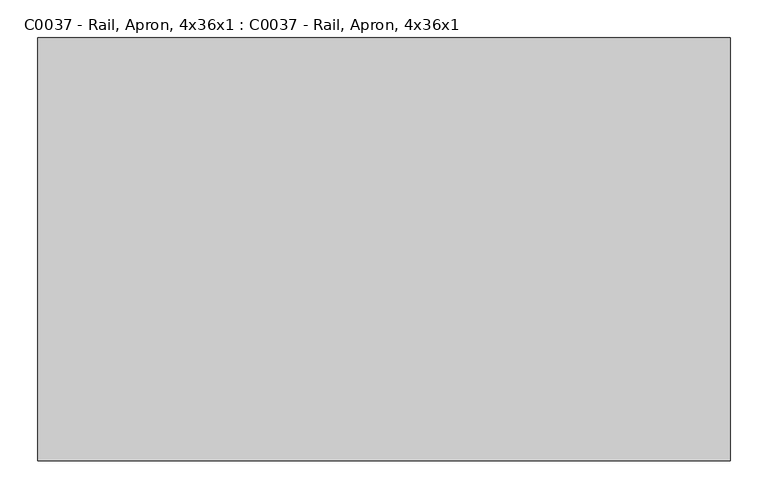
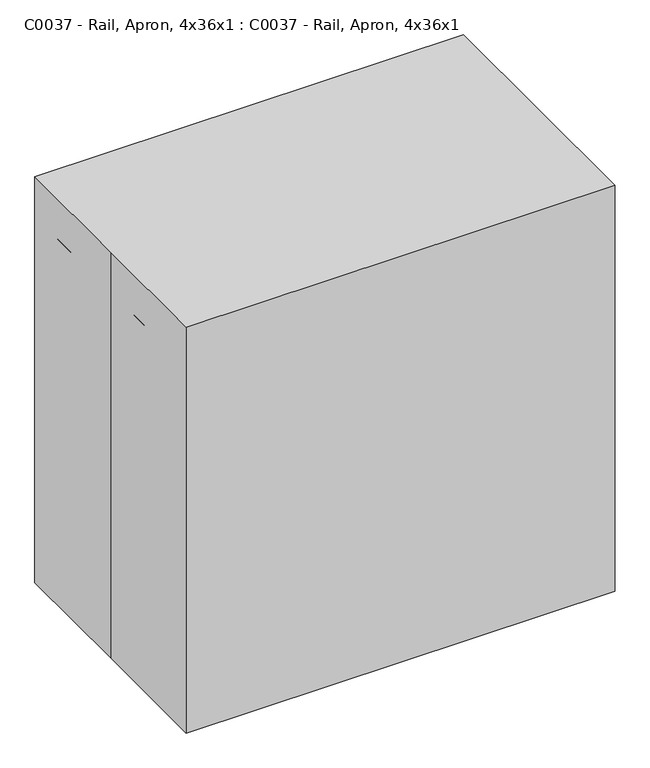
"""IFC4 building model written with IfcOpenShell, lengths in millimetres: proxy geometry, C0037 - Rail, Apron, 4x36x1 : C0037 - Rail, Apron, 4x36x1."""

from ifc_helpers import new_model, si_unit, frame, origin, origin_with_axes, place, context, project, spatial, polyline, outline, extrude, source, transform, mapped, element, save


def c0037_rail_apron_4x36x1_c0037_rail_apron_4x36x1_112512d8(model_context):
    return source(origin(), model_context, "Body", "SweptSolid", [
        extrude(outline(polyline([(-457.2, 279.4), (457.2, 279.4), (457.2, -279.4), (-457.2, -279.4), (-457.2, 0.0), (-457.2, 279.4)])), origin_with_axes(), (0.0, 0.0, 1.0), 914.4),
        extrude(outline(polyline([(438.15, -260.35), (438.15, 279.4), (457.2, 279.4), (457.2, -260.35), (438.15, -260.35)])), frame((0.0, 0.0, 673.0674767), z_axis=(0.0, 0.0, 1.0), x_axis=(1.0, 0.0, 0.0)), (0.0, 0.0, 1.0), 152.4),
        extrude(outline(polyline([(-457.2, -260.35), (-457.2, 279.4), (-438.15, 279.4), (-438.15, -260.35), (-457.2, -260.35)])), frame((0.0, 0.0, 673.0674767), z_axis=(0.0, 0.0, 1.0), x_axis=(1.0, 0.0, 0.0)), (0.0, 0.0, 1.0), 152.4),
        extrude(outline(polyline([(457.2, -279.4), (-457.2, -279.4), (-457.2, -260.35), (457.2, -260.35), (457.2, -279.4)])), frame((0.0, 0.0, 673.0674767), z_axis=(0.0, 0.0, 1.0), x_axis=(1.0, 0.0, 0.0)), (0.0, 0.0, 1.0), 152.4),
        extrude(outline(polyline([(438.15, 260.35), (-438.15, 260.35), (-438.15, 279.4), (438.15, 279.4), (438.15, 260.35)])), frame((0.0, 0.0, 673.0674767), z_axis=(0.0, 0.0, 1.0), x_axis=(1.0, 0.0, 0.0)), (0.0, 0.0, 1.0), 133.35),
    ])


if __name__ == "__main__":
    model = new_model("IFC4")
    model_context = context("Model", 3, world=origin())
    ifc_project = project(units=[si_unit("LENGTHUNIT", "METRE", prefix="MILLI")], contexts=[model_context])
    site = spatial("IfcSite", under=ifc_project)
    building = spatial("IfcBuilding", under=site)
    placement = place(None, origin())
    c0037_rail_apron_4x36x1_c0037_rail_apron_4x36x1_shape = c0037_rail_apron_4x36x1_c0037_rail_apron_4x36x1_112512d8(model_context)
    element("IfcBuildingElementProxy", 1, Name="C0037 - Rail, Apron, 4x36x1 : C0037 - Rail, Apron, 4x36x1", ObjectType="C0037 - Rail, Apron, 4x36x1 : C0037 - Rail, Apron, 4x36x1", at=placement, inside=building, context=model_context, shape_type="MappedRepresentation", body=[
        mapped(c0037_rail_apron_4x36x1_c0037_rail_apron_4x36x1_shape, transform((0.0, 0.0, 0.0), x_axis=(1.0, 0.0, 0.0), y_axis=(0.0, 1.0, 0.0), z_axis=(0.0, 0.0, 1.0))),
    ])
    save(model, "model.ifc")

# Revit data of these elements
# Project information
#   Sheets - Total = "6"
#   Project Issue Date = "Issue Date"
#   Project Status = "Project Status"
#   Client Name = "Owner"
#   Project Address = "Enter address here"
#   Project Name = "Project Name"
#   Project Number = "Project Number"
#   Publication Date = "30-Jan-15"
# Type "C0037 - Rail, Apron, 4x36x1 : C0037 - Rail, Apron, 4x36x1"
#   Watts2 = "0"
#   Watts1 = "0"
#   Unit_Issue = "EA"
#   UTIL_6_Misc = "-"
#   UTIL_5_NonMedGas = "-"
#   UTIL_4_MiscGas = "-"
#   UTIL_3_MedGas = "-"
#   UTIL_2_Elec = "-"
#   UTIL_1_WaterDrain = "-"
#   Nomenclature = "Rail, Apron, 4x36x1"
#   NSN = "6530"
#   Location [instance default] = ""
#   JSN = "C0037"
#   Fund_Source_VA = "-"
#   Fund_Source_Navy = "-"
#   Fund_Source_Army = "-"
#   Fund_Source_AF = "-"
#   ELEC_Volts2 = "0"
#   ELEC_Volts1 = "0"
#   ELEC_Phase2 = "0"
#   ELEC_Phase1 = "0"
#   ELEC_HertzSwitch = "0"
#   ELEC_HertzDependent = "0"
#   ELEC_Hertz = "0"
#   ELEC_Amps2 = "0"
#   ELEC_Amps1 = "0"
#   DetailDescription = "Apron rail. Also referred to as an apron front, apron panel, or knee space rail. Used to close in front knee space area and/or provide work surface support between two base cabinets or a base cabinet and wall. Apron rails should be ordered in pairs to provide both front and rear work surface support."
#   CAT_VA = "A"
#   CAT_Navy = "A"
#   CAT_IHS = "-"
#   CAT_Army = "A"
#   CAT_AF = "A"
#   BTUperhour = "0"
#   Weight_IP = 10
#   DIM_Width_IP = 3' - 0"
#   DIM_Height_IP = 3' - 0"
#   DIM_Depth_IP = 1' - 10"
#   Top Panel Material = none
#   Toe Panel Material = none
#   Side Panel Material = none
#   Shelf Panel Material = none
#   Drawer Front Material = none
#   Door Panel Material = none
#   Back Panel Material = none
#   Assembly Code = ""
# Element 1 (IfcBuildingElementProxy, "C0037 - Rail, Apron, 4x36x1 : C0037 - Rail, Apron, 4x36x1")
#   Materials on its faces: "EquipSpace"
# Materials
#   "EquipSpace": class "Unassigned", colour RGB 221 217 195, transparency 0.5
